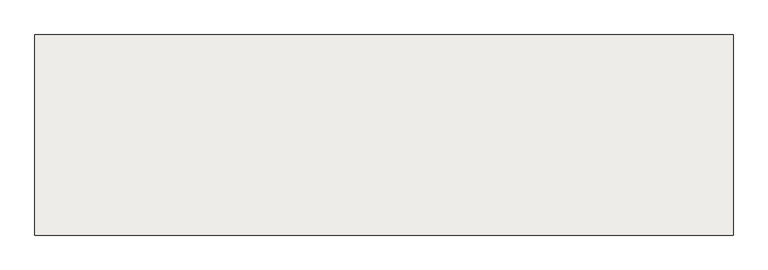
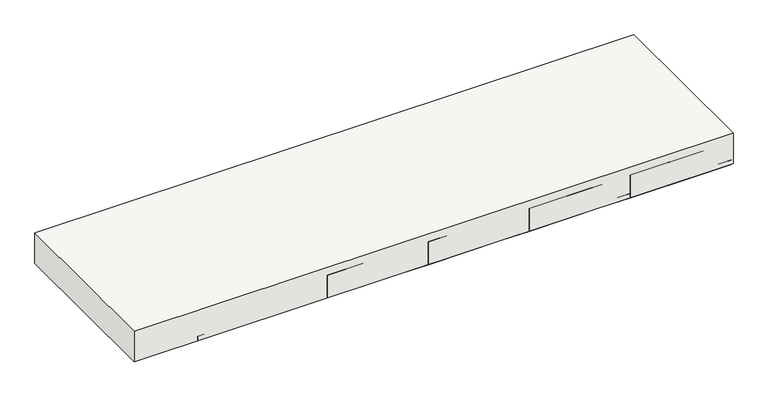
"""IFC4 building model written with IfcOpenShell, lengths in millimetres: slab geometry, Pano 18 (16 cm)."""

from ifc_helpers import new_model, si_unit, origin, origin_with_axes, place, context, project, spatial, polyline, outline, extrude, source, transform, mapped, element, save


def slab_06c70554(model_context):
    return source(origin(), model_context, "Body", "SweptSolid", [
        extrude(outline(polyline([(5760.0, 5350.0), (5760.0, 4500.0), (2795.0, 4500.0), (2795.0, 5350.0), (5760.0, 5350.0)])), origin_with_axes(), (0.0, 0.0, 1.0), 160.0),
        extrude(outline(polyline([(5610.0, 4500.0), (5250.0, 4500.0), (5250.0, 4995.0), (5610.0, 4995.0), (5610.0, 4500.0)])), origin_with_axes(), (0.0, 0.0, 1.0), 120.0),
        extrude(outline(polyline([(3250.0, 4500.0), (3110.0, 4500.0), (3110.0, 5350.0), (3250.0, 5350.0), (3250.0, 4500.0)])), origin_with_axes(), (0.0, 0.0, 1.0), 24.0),
        extrude(outline(polyline([(4750.0, 4500.0), (4610.0, 4500.0), (4610.0, 5350.0), (4750.0, 5350.0), (4750.0, 4500.0)])), origin_with_axes(), (0.0, 0.0, 1.0), 24.0),
        extrude(outline(polyline([(3610.0, 4500.0), (3250.0, 4500.0), (3250.0, 4995.0), (3610.0, 4995.0), (3610.0, 4500.0)])), origin_with_axes(), (0.0, 0.0, 1.0), 120.0),
        extrude(outline(polyline([(3610.0, 5000.0), (3250.0, 5000.0), (3250.0, 5345.0), (3610.0, 5345.0), (3610.0, 5000.0)])), origin_with_axes(), (0.0, 0.0, 1.0), 120.0),
        extrude(outline(polyline([(5750.0, 4500.0), (5610.0, 4500.0), (5610.0, 5350.0), (5750.0, 5350.0), (5750.0, 4500.0)])), origin_with_axes(), (0.0, 0.0, 1.0), 24.0),
        extrude(outline(polyline([(5610.0, 5000.0), (5250.0, 5000.0), (5250.0, 5345.0), (5610.0, 5345.0), (5610.0, 5000.0)])), origin_with_axes(), (0.0, 0.0, 1.0), 120.0),
        extrude(outline(polyline([(4610.0, 5000.0), (4250.0, 5000.0), (4250.0, 5345.0), (4610.0, 5345.0), (4610.0, 5000.0)])), origin_with_axes(), (0.0, 0.0, 1.0), 120.0),
        extrude(outline(polyline([(5110.0, 5000.0), (4750.0, 5000.0), (4750.0, 5345.0), (5110.0, 5345.0), (5110.0, 5000.0)])), origin_with_axes(), (0.0, 0.0, 1.0), 120.0),
        extrude(outline(polyline([(4610.0, 4500.0), (4250.0, 4500.0), (4250.0, 4995.0), (4610.0, 4995.0), (4610.0, 4500.0)])), origin_with_axes(), (0.0, 0.0, 1.0), 120.0),
        extrude(outline(polyline([(3750.0, 4500.0), (3610.0, 4500.0), (3610.0, 5350.0), (3750.0, 5350.0), (3750.0, 4500.0)])), origin_with_axes(), (0.0, 0.0, 1.0), 24.0),
        extrude(outline(polyline([(5250.0, 4500.0), (5110.0, 4500.0), (5110.0, 5350.0), (5250.0, 5350.0), (5250.0, 4500.0)])), origin_with_axes(), (0.0, 0.0, 1.0), 24.0),
        extrude(outline(polyline([(4110.0, 5000.0), (3750.0, 5000.0), (3750.0, 5345.0), (4110.0, 5345.0), (4110.0, 5000.0)])), origin_with_axes(), (0.0, 0.0, 1.0), 120.0),
        extrude(outline(polyline([(5110.0, 4500.0), (4750.0, 4500.0), (4750.0, 4995.0), (5110.0, 4995.0), (5110.0, 4500.0)])), origin_with_axes(), (0.0, 0.0, 1.0), 120.0),
        extrude(outline(polyline([(4250.0, 4500.0), (4110.0, 4500.0), (4110.0, 5350.0), (4250.0, 5350.0), (4250.0, 4500.0)])), origin_with_axes(), (0.0, 0.0, 1.0), 24.0),
        extrude(outline(polyline([(4110.0, 4500.0), (3750.0, 4500.0), (3750.0, 4995.0), (4110.0, 4995.0), (4110.0, 4500.0)])), origin_with_axes(), (0.0, 0.0, 1.0), 120.0),
    ])


if __name__ == "__main__":
    model = new_model("IFC4")
    model_context = context("Model", 3, world=origin())
    ifc_project = project(units=[si_unit("LENGTHUNIT", "METRE", prefix="MILLI")], contexts=[model_context])
    site = spatial("IfcSite", under=ifc_project)
    building = spatial("IfcBuilding", under=site)
    placement = place(None, origin())
    slab_shape = slab_06c70554(model_context)
    element("IfcSlab", 1, ObjectType="Pano 18 (16 cm)", at=placement, inside=building, context=model_context, shape_type="MappedRepresentation", body=[
        mapped(slab_shape, transform((0.0, 0.0, 0.0), x_axis=(1.0, 0.0, 0.0), y_axis=(0.0, 1.0, 0.0), z_axis=(0.0, 0.0, 1.0))),
    ])
    save(model, "model.ifc")

# Revit data of these elements
# Element 1 (IfcSlab, "Pano 18 (16 cm)")
#   Materials on its faces: "Molde de poliestireno", "Concreto armado", "RGB 168-169-158"
# Materials
#   "Molde de poliestireno": class "Não atribuído", colour RGB 255 255 255, transparency 0
#   "Concreto armado": class "Não atribuído", colour RGB 168 169 158, transparency 0
#   "RGB 168-169-158": class "Não atribuído", colour RGB 168 169 158, transparency 0
